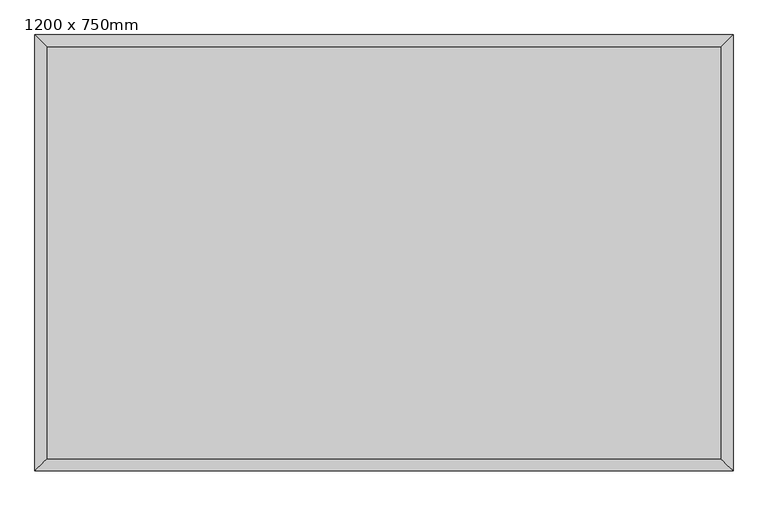
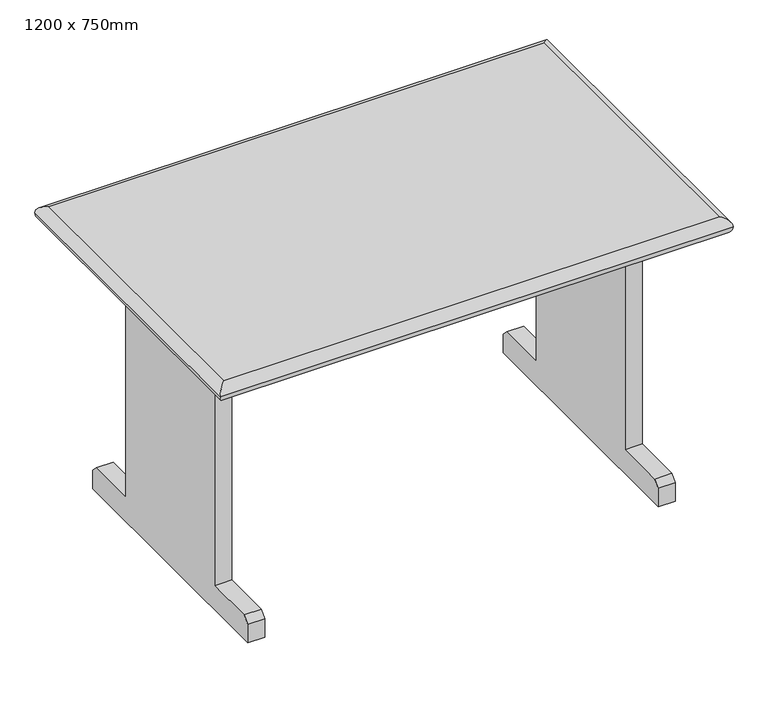
"""IFC4 building model written with IfcOpenShell, lengths in millimetres: furniture geometry, ダイニングテーブル : 1200 x 750mm."""

from ifc_helpers import new_model, si_unit, frame, origin, place, context, project, spatial, polyline, ellipse_curve, outline, extrude, source, transform, mapped, element, save
from ifc_brep_helpers import plane_surface, cylinder_surface, advanced_brep


def furniture_1200_x_750mm_ce0cf10f(model_context):
    return source(origin(), model_context, "Body", "SolidModel", [
        advanced_brep(
        [(600.0, 375.0, 680.0), (580.0, 355.0, 700.0), (580.0, -355.0, 700.0), (600.0, -375.0, 680.0), (580.0, -355.0, 660.0), (580.0, 355.0, 660.0), (-580.0, -355.0, 700.0), (-600.0, -375.0, 680.0), (-580.0, -355.0, 660.0), (-580.0, 355.0, 700.0), (-600.0, 375.0, 680.0), (-580.0, 355.0, 660.0)],
        [
            (0, 1, ellipse_curve(frame((580.0, 355.0, 680.0), z_axis=(0.7071067811865475, -0.7071067811865475, 0.0), x_axis=(0.7071067811865474, 0.7071067811865476, 0.0)), 28.2842712, 20.0)),
            (1, 2),
            (2, 3, ellipse_curve(frame((580.0, -355.0, 680.0), z_axis=(0.7071067811865475, 0.7071067811865475, 0.0), x_axis=(-0.7071067811865474, 0.7071067811865476, 0.0)), 28.2842712, 20.0)),
            (3, 0),
            (3, 4, ellipse_curve(frame((580.0, -355.0, 680.0), z_axis=(0.7071067811865475, 0.7071067811865475, 0.0), x_axis=(-0.7071067811865474, 0.7071067811865476, 0.0)), 28.2842712, 20.0)),
            (4, 5),
            (5, 0, ellipse_curve(frame((580.0, 355.0, 680.0), z_axis=(0.7071067811865475, -0.7071067811865475, 0.0), x_axis=(0.7071067811865474, 0.7071067811865476, 0.0)), 28.2842712, 20.0)),
            (2, 6),
            (6, 7, ellipse_curve(frame((-580.0, -355.0, 680.0), z_axis=(0.7071067811865475, -0.7071067811865475, 0.0), x_axis=(0.7071067811865476, 0.7071067811865474, 0.0)), 28.2842712, 20.0)),
            (7, 3),
            (7, 8, ellipse_curve(frame((-580.0, -355.0, 680.0), z_axis=(0.7071067811865475, -0.7071067811865475, 0.0), x_axis=(0.7071067811865476, 0.7071067811865474, 0.0)), 28.2842712, 20.0)),
            (8, 4),
            (6, 9),
            (9, 10, ellipse_curve(frame((-580.0, 355.0, 680.0), z_axis=(-0.7071067811865475, -0.7071067811865475, 0.0), x_axis=(0.7071067811865474, -0.7071067811865476, 0.0)), 28.2842712, 20.0)),
            (10, 7),
            (10, 11, ellipse_curve(frame((-580.0, 355.0, 680.0), z_axis=(-0.7071067811865475, -0.7071067811865475, 0.0), x_axis=(0.7071067811865474, -0.7071067811865476, 0.0)), 28.2842712, 20.0)),
            (11, 8),
            (0, 10),
            (9, 1),
            (5, 11),
        ],
        [
            cylinder_surface(frame((580.0, 355.0, 680.0), z_axis=(0.0, 1.0, 0.0), x_axis=(1.0, 0.0, 0.0)), 20.0),
            cylinder_surface(frame((580.0, -355.0, 680.0), z_axis=(1.0, 0.0, 0.0), x_axis=(0.0, -1.0, 0.0)), 20.0),
            cylinder_surface(frame((-580.0, -355.0, 680.0), z_axis=(0.0, -1.0, 0.0), x_axis=(-1.0, 0.0, 0.0)), 20.0),
            cylinder_surface(frame((-580.0, 355.0, 680.0), z_axis=(-1.0, 0.0, 0.0), x_axis=(0.0, 1.0, 0.0)), 20.0),
            plane_surface(frame((-580.0, 355.0, 700.0), z_axis=(0.0, 0.0, 1.0), x_axis=(-1.0, 0.0, 0.0))),
            plane_surface(frame((-580.0, 355.0, 660.0), z_axis=(0.0, 0.0, -1.0), x_axis=(1.0, 0.0, 0.0))),
        ],
        [
            (0, [[1, 2, 3, 4]]),
            (0, [[-4, 5, 6, 7]]),
            (1, [[-3, 8, 9, 10]]),
            (1, [[-5, -10, 11, 12]]),
            (2, [[-9, 13, 14, 15]]),
            (2, [[-11, -15, 16, 17]]),
            (3, [[-1, 18, -14, 19]]),
            (3, [[-7, 20, -16, -18]]),
            (4, [[-2, -19, -13, -8]]),
            (5, [[-6, -12, -17, -20]]),
        ],
    ),
        extrude(outline(polyline([(-180.0, 660.0), (0.0, 660.0), (180.0, 660.0), (180.0, 60.0), (300.0, 60.0), (314.1421356, 45.8578644), (314.1421356, 0.0), (0.0, 0.0), (-314.1421356, 0.0), (-314.1421356, 45.8578644), (-300.0, 60.0), (-180.0, 60.0), (-180.0, 660.0)])), frame((460.0, 0.0, 0.0), z_axis=(1.0, 0.0, 0.0), x_axis=(0.0, 1.0, 0.0)), (0.0, 0.0, 1.0), 40.0),
        extrude(outline(polyline([(-180.0, 660.0), (0.0, 660.0), (180.0, 660.0), (180.0, 60.0), (300.0, 60.0), (314.1421356, 45.8578644), (314.1421356, 0.0), (0.0, 0.0), (-314.1421356, 0.0), (-314.1421356, 45.8578644), (-300.0, 60.0), (-180.0, 60.0), (-180.0, 660.0)])), frame((-500.0, 0.0, 0.0), z_axis=(1.0, 0.0, 0.0), x_axis=(0.0, 1.0, 0.0)), (0.0, 0.0, 1.0), 40.0),
    ])


if __name__ == "__main__":
    model = new_model("IFC4")
    model_context = context("Model", 3, world=origin())
    ifc_project = project(units=[si_unit("LENGTHUNIT", "METRE", prefix="MILLI")], contexts=[model_context])
    site = spatial("IfcSite", under=ifc_project)
    building = spatial("IfcBuilding", under=site)
    placement = place(None, origin())
    furniture_1200_x_750mm_shape = furniture_1200_x_750mm_ce0cf10f(model_context)
    element("IfcFurniture", 1, ObjectType="ダイニングテーブル : 1200 x 750mm", at=placement, inside=building, context=model_context, shape_type="MappedRepresentation", body=[
        mapped(furniture_1200_x_750mm_shape, transform((0.0, 0.0, 0.0), x_axis=(1.0, 0.0, 0.0), y_axis=(0.0, 1.0, 0.0), z_axis=(0.0, 0.0, 1.0))),
    ])
    save(model, "model.ifc")

# Revit data of these elements
# Type "ダイニングテーブル : 1200 x 750mm"
#   Keynote = "12490.BB1"
#   幅 = 1200 mm
#   奥行き = 750 mm
#   本体 = 木目 - ナチュラル
#   Default Elevation = 0
# Element 1 (IfcFurniture, "ダイニングテーブル : 1200 x 750mm")
#   Materials on its faces: "木目 - ナチュラル"
# Materials
#   "木目 - ナチュラル": class "木材", colour RGB 204 173 122, transparency 0, Cost = 0
